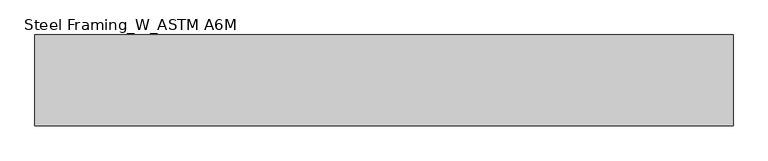
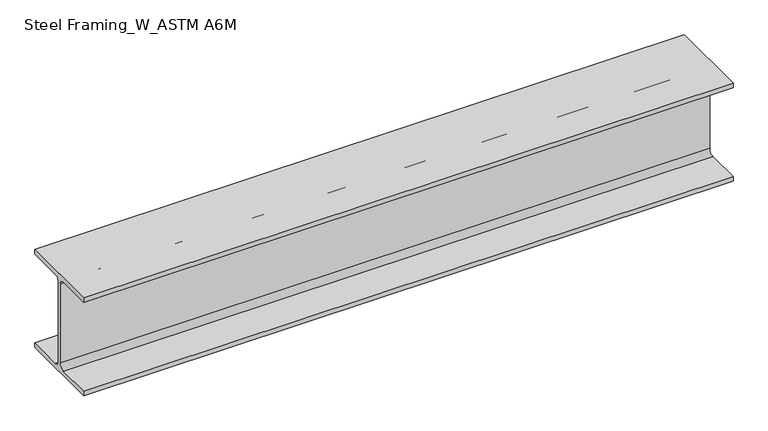
"""IFC4 building model written with IfcOpenShell, lengths in millimetres: beam geometry, Steel Framing_W_ASTM A6M : H_SB_AR_S02_W250x49.1_G5."""

import ifcopenshell
import ifcopenshell.guid

model = None  # the IFC model being written
_history = None  # IfcOwnerHistory: only IFC2X3 demands one
_inside = {}  # id of a spatial element -> (the spatial element, [elements in it])
_under = {}  # id of a project, library or spatial element -> (it, [spatial elements below it])
_declared = {}  # id of a project -> (the project, [libraries it declares])
_typed = {}  # id of a type object -> (the type object, [elements of that type])
_made_of = {}  # id of a material, layer set ... -> (it, [elements and type objects made of it])


def new_model(schema):
    """Start an empty IFC model of exactly this schema.

    Asked for "IFC4X3", IfcOpenShell would pick the latest addendum, in which some entities
    have other attributes; the version numbers below select the first issue.
    IFC2X3 requires an IfcOwnerHistory on every rooted entity: one is made here for all.
    """
    global model, _history
    if schema == "IFC4X3":
        model = ifcopenshell.file(schema_version=(4, 3, 0, 0))
    else:
        model = ifcopenshell.file(schema=schema)
    _inside.clear()
    _under.clear()
    _declared.clear()
    _typed.clear()
    _made_of.clear()
    _history = None
    if model.schema == "IFC2X3":
        org = make("IfcOrganization", Name="unknown")
        user = make(
            "IfcPersonAndOrganization",
            ThePerson=make("IfcPerson", FamilyName="unknown"),
            TheOrganization=org,
        )
        app = make(
            "IfcApplication",
            ApplicationDeveloper=org,
            Version="unknown",
            ApplicationFullName="unknown",
            ApplicationIdentifier="unknown",
        )
        _history = make(
            "IfcOwnerHistory",
            OwningUser=user,
            OwningApplication=app,
            ChangeAction="ADDED",
            CreationDate=0,
        )
    return model


def make(cls, **values):
    """One entity of the class cls with the attributes given. An attribute that is None is left unset."""
    return model.create_entity(
        cls, **{name: value for name, value in values.items() if value is not None}
    )


def rooted(cls, **values):
    """An entity with a GlobalId (a new one), such as an element, a storey or a relation."""
    return make(cls, GlobalId=ifcopenshell.guid.new(), OwnerHistory=_history, **values)


def si_unit(unit_type, name, prefix=None):
    """IfcSIUnit, for example si_unit("LENGTHUNIT", "METRE", prefix="MILLI")."""
    return make("IfcSIUnit", UnitType=unit_type, Prefix=prefix, Name=name)


def assignment(units):
    """IfcUnitAssignment: the units of a project."""
    return None if units is None else make("IfcUnitAssignment", Units=units)


def point(xyz):
    """IfcCartesianPoint."""
    return None if xyz is None else make("IfcCartesianPoint", Coordinates=xyz)


def direction(xyz):
    """IfcDirection."""
    return None if xyz is None else make("IfcDirection", DirectionRatios=xyz)


def frame(location, z_axis=None, x_axis=None):
    """IfcAxis2Placement3D, a coordinate frame: its origin and axes. An axis left out is left unset."""
    return make(
        "IfcAxis2Placement3D",
        Location=point(location),
        Axis=direction(z_axis),
        RefDirection=direction(x_axis),
    )


def frame_2d(location, x_axis=None):
    """IfcAxis2Placement2D, a coordinate frame in the plane: its origin and x axis."""
    return make(
        "IfcAxis2Placement2D", Location=point(location), RefDirection=direction(x_axis)
    )


def origin():
    """The frame at (0, 0, 0) with its axes left unset."""
    return frame((0.0, 0.0, 0.0))


def place(relative_to, where):
    """IfcLocalPlacement: puts the frame where relative to a parent placement (None: the world)."""
    return make(
        "IfcLocalPlacement", PlacementRelTo=relative_to, RelativePlacement=where
    )


def context(
    kind, dimensions, precision=None, world=None, true_north=None, identifier=None
):
    """IfcGeometricRepresentationContext, for example the 3D "Model" context."""
    return make(
        "IfcGeometricRepresentationContext",
        ContextIdentifier=identifier,
        ContextType=kind,
        CoordinateSpaceDimension=dimensions,
        Precision=precision,
        WorldCoordinateSystem=world,
        TrueNorth=true_north,
    )


def project(units=None, contexts=None):
    """IfcProject with its units and contexts."""
    return rooted(
        "IfcProject",
        Name="project",
        RepresentationContexts=contexts,
        UnitsInContext=assignment(units),
    )


def spatial(cls, under=None, at=None, **own):
    """A site, building, storey or space (cls), placed at a placement, below another one or the project."""
    s = rooted(cls, ObjectPlacement=at, **own)
    if under is not None:
        _under.setdefault(under.id(), (under, []))[1].append(s)
    return s


def polyline(points):
    """IfcPolyline through the points."""
    return make("IfcPolyline", Points=[point(p) for p in points])


def circle_curve(where, radius):
    """IfcCircle in the frame where."""
    return make("IfcCircle", Position=where, Radius=radius)


def trimmed(basis, trim1, trim2, sense, master):
    """IfcTrimmedCurve: the piece of a basis curve between two trims."""
    return make(
        "IfcTrimmedCurve",
        BasisCurve=basis,
        Trim1=trim1,
        Trim2=trim2,
        SenseAgreement=sense,
        MasterRepresentation=master,
    )


def segment(curve, same_sense, transition):
    """IfcCompositeCurveSegment."""
    return make(
        "IfcCompositeCurveSegment",
        Transition=transition,
        SameSense=same_sense,
        ParentCurve=curve,
    )


def composite_curve(segments, self_intersect=None):
    """IfcCompositeCurve: segments joined end to end."""
    return make("IfcCompositeCurve", Segments=segments, SelfIntersect=self_intersect)


def outline(outer, holes=None, kind="AREA"):
    """IfcArbitraryClosedProfileDef: a profile drawn as a closed curve; with holes, ...WithVoids."""
    if holes is None:
        return make("IfcArbitraryClosedProfileDef", ProfileType=kind, OuterCurve=outer)
    return make(
        "IfcArbitraryProfileDefWithVoids",
        ProfileType=kind,
        OuterCurve=outer,
        InnerCurves=holes,
    )


def extrude(swept, where, along, depth):
    """IfcExtrudedAreaSolid: the profile swept, set in the frame where, extruded along a direction by depth."""
    return make(
        "IfcExtrudedAreaSolid",
        SweptArea=swept,
        Position=where,
        ExtrudedDirection=direction(along),
        Depth=depth,
    )


def shape(context_of_items, identifier, shape_type, items):
    """IfcShapeRepresentation: the items that make up one representation, for example the "Body"."""
    return make(
        "IfcShapeRepresentation",
        ContextOfItems=context_of_items,
        RepresentationIdentifier=identifier,
        RepresentationType=shape_type,
        Items=items,
    )


def source(mapping_origin, context_of_items, identifier, shape_type, items):
    """IfcRepresentationMap: a shape defined once, which mapped items show again and again."""
    return make(
        "IfcRepresentationMap",
        MappingOrigin=mapping_origin,
        MappedRepresentation=shape(context_of_items, identifier, shape_type, items),
    )


def transform(
    local_origin,
    x_axis=None,
    y_axis=None,
    z_axis=None,
    scale=None,
    scale2=None,
    scale3=None,
    uniform=True,
):
    """IfcCartesianTransformationOperator3D, or its non-uniform kind. x_axis, y_axis, z_axis: its Axis1, 2, 3."""
    if uniform:
        return make(
            "IfcCartesianTransformationOperator3D",
            Axis1=direction(x_axis),
            Axis2=direction(y_axis),
            LocalOrigin=point(local_origin),
            Scale=scale,
            Axis3=direction(z_axis),
        )
    return make(
        "IfcCartesianTransformationOperator3DnonUniform",
        Axis1=direction(x_axis),
        Axis2=direction(y_axis),
        LocalOrigin=point(local_origin),
        Scale=scale,
        Axis3=direction(z_axis),
        Scale2=scale2,
        Scale3=scale3,
    )


def mapped(mapping_source, mapping_target):
    """IfcMappedItem: shows the shape of a source again, moved by a transform."""
    return make(
        "IfcMappedItem", MappingSource=mapping_source, MappingTarget=mapping_target
    )


def made_of(thing, what):
    """Note that an element or type object is made of a material, layer set ...; save() writes the relation."""
    if what is not None:
        _made_of.setdefault(what.id(), (what, []))[1].append(thing)
    return thing


def element(
    cls,
    number,
    at=None,
    inside=None,
    cuts=None,
    type_object=None,
    material=None,
    context=None,
    identifier="Body",
    shape_type=None,
    held_by="IfcProductDefinitionShape",
    body=None,
    shapes=None,
    **own,
):
    """One element of the class cls, such as IfcWall. Its Tag is "e" and its number.

    at: its placement. inside: the storey or other place that contains it. cuts: it is an
    opening in that element (IfcRelVoidsElement). A single representation is given by context,
    identifier, shape_type and body (its items); several are given by shapes. held_by: the class
    of the entity that holds the representations. save() writes the other relations.
    """
    e = rooted(cls, Tag="e%d" % number, ObjectPlacement=at, **own)
    if body is not None:
        shapes = [shape(context, identifier, shape_type, body)]
    if shapes is not None:
        e.Representation = make(held_by, Representations=shapes)
    if inside is not None:
        _inside.setdefault(inside.id(), (inside, []))[1].append(e)
    if cuts is not None:
        rooted(
            "IfcRelVoidsElement", RelatingBuildingElement=cuts, RelatedOpeningElement=e
        )
    if type_object is not None:
        _typed.setdefault(type_object.id(), (type_object, []))[1].append(e)
    return made_of(e, material)


def aggregate(whole, parts):
    """IfcRelAggregates: a whole, such as a stair, and the parts it consists of."""
    return rooted("IfcRelAggregates", RelatingObject=whole, RelatedObjects=parts)


def save(model, path):
    """Write the relations noted so far, then the file.

    IfcRelAggregates (storeys below a building ...), IfcRelContainedInSpatialStructure (elements
    in a storey), IfcRelDefinesByType, IfcRelAssociatesMaterial and IfcRelDeclares: one each for
    every whole, place, type object, material and project.
    """
    for whole, parts in _under.values():
        aggregate(whole, parts)
    for where, things in _inside.values():
        rooted(
            "IfcRelContainedInSpatialStructure",
            RelatedElements=things,
            RelatingStructure=where,
        )
    for kind, things in _typed.values():
        rooted("IfcRelDefinesByType", RelatedObjects=things, RelatingType=kind)
    for what, things in _made_of.values():
        rooted("IfcRelAssociatesMaterial", RelatedObjects=things, RelatingMaterial=what)
    for by, libraries in _declared.values():
        rooted("IfcRelDeclares", RelatingContext=by, RelatedDefinitions=libraries)
    model.write(path)


def steel_framing_w_astm_a6m_56f27783(model_context):
    return source(origin(), model_context, "Body", "SweptSolid", [
        extrude(outline(composite_curve([segment(polyline([(101.0, -112.5), (101.0, -123.5), (-101.0, -123.5), (-101.0, -112.5), (-16.385, -112.5)]), True, "CONTINUOUS"), segment(trimmed(circle_curve(frame_2d((-16.385, -99.8)), 12.7), [point((-16.385, -112.5))], [point((-3.685, -99.8))], True, "CARTESIAN"), True, "CONTINUOUS"), segment(polyline([(-3.685, -99.8), (-3.685, 99.8)]), True, "CONTINUOUS"), segment(trimmed(circle_curve(frame_2d((-16.385, 99.8)), 12.7), [point((-3.685, 99.8))], [point((-16.385, 112.5))], True, "CARTESIAN"), True, "CONTINUOUS"), segment(polyline([(-16.385, 112.5), (-101.0, 112.5), (-101.0, 123.5), (101.0, 123.5), (101.0, 112.5), (16.385, 112.5)]), True, "CONTINUOUS"), segment(trimmed(circle_curve(frame_2d((16.385, 99.8)), 12.7), [point((16.385, 112.5))], [point((3.685, 99.8))], True, "CARTESIAN"), True, "CONTINUOUS"), segment(polyline([(3.685, 99.8), (3.685, -99.8)]), True, "CONTINUOUS"), segment(trimmed(circle_curve(frame_2d((16.385, -99.8)), 12.7), [point((3.685, -99.8))], [point((16.385, -112.5))], True, "CARTESIAN"), True, "CONTINUOUS"), segment(polyline([(16.385, -112.5), (101.0, -112.5)]), True, "CONTINUOUS")], self_intersect=False)), frame((-684.3, 0.0, 0.0), z_axis=(1.0, 0.0, 0.0), x_axis=(0.0, 1.0, 0.0)), (0.0, 0.0, 1.0), 1551.3),
    ])


if __name__ == "__main__":
    model = new_model("IFC4")
    model_context = context("Model", 3, world=origin())
    ifc_project = project(units=[si_unit("LENGTHUNIT", "METRE", prefix="MILLI")], contexts=[model_context])
    site = spatial("IfcSite", under=ifc_project)
    building = spatial("IfcBuilding", under=site)
    placement = place(None, origin())
    steel_framing_w_astm_a6m_shape = steel_framing_w_astm_a6m_56f27783(model_context)
    element("IfcBeam", 1, ObjectType="Steel Framing_W_ASTM A6M : H_SB_AR_S02_W250x49.1_G5", at=placement, inside=building, context=model_context, shape_type="MappedRepresentation", body=[
        mapped(steel_framing_w_astm_a6m_shape, transform((0.0, 0.0, 0.0), x_axis=(1.0, 0.0, 0.0), y_axis=(0.0, 1.0, 0.0), z_axis=(0.0, 0.0, 1.0))),
    ])
    save(model, "model.ifc")

# Revit data of these elements
# Type "Steel Framing_W_ASTM A6M : H_SB_AR_S02_W250x49.1_G5"
#   Type Mark = "G5"
#   Section Name Key = "W10x33"
#   Width = 20.2 cm
#   Web Thickness = 0.737 cm
#   Web Fillet = 1.27 cm
#   Warping Constant = 212000.0 cm⁶
#   Torsional Moment of Inertia = 24.30 cm⁴
#   Section Area = 62.6 cm²
#   Plastic Modulus weak axis = 229.0 cm³
#   Plastic Modulus strong axis = 636.0 cm³
#   Perimeter = 1.27 m²/m
#   Nominal Weight = 49.10 kgf/m
#   Moment of Inertia weak axis = 1520.00 cm⁴
#   Moment of Inertia strong axis = 7120.00 cm⁴
#   Height = 24.7 cm
#   Flange Thickness = 1.1 cm
#   Elastic Modulus weak axis = 151.0 cm³
#   Elastic Modulus strong axis = 574.0 cm³
#   Centroid Vertical = 12.35 cm
#   Centroid Horizontal = 10.1 cm
#   Length [instance default] = 1500 mm
#   Structural Material [instance default] = Steel, 45-345
#   Bolt Spacing = 0
#   Assembly Code = ""
# Element 1 (IfcBeam, "Steel Framing_W_ASTM A6M : H_SB_AR_S02_W250x49.1_G5")
#   Materials on its faces: "Steel, 45-345"
# Materials
#   "Steel, 45-345": class "Metal", colour RGB 189 187 185, transparency 0, Description = "Steel 345 MPa", Cost = 0
